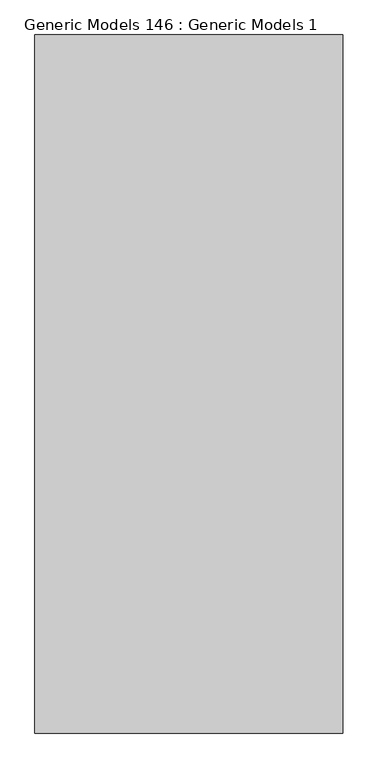
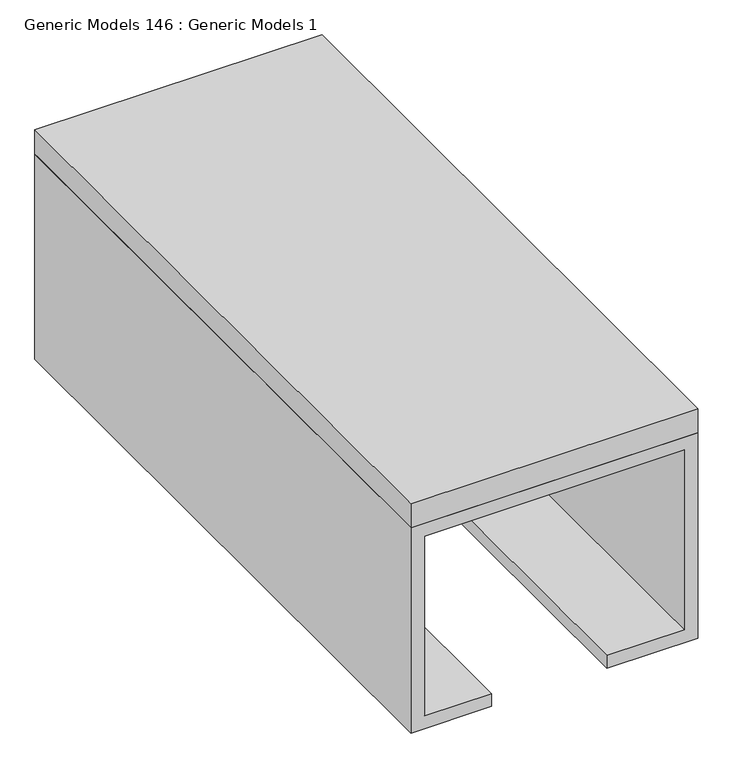
"""IFC4 building model written with IfcOpenShell, lengths in millimetres: proxy geometry, Generic Models 146 : Generic Models 1."""

from ifc_helpers import new_model, si_unit, frame, origin, place, context, project, spatial, polyline, outline, extrude, source, transform, mapped, element, save


def generic_models_146_generic_models_1_9775dfd0(model_context):
    return source(origin(), model_context, "Body", "SweptSolid", [
        extrude(outline(polyline([(51176.9547769, 0.0), (50639.5319345, 0.0), (50639.5319345, 1219.2), (51176.9547769, 1219.2), (51176.9547769, 0.0)])), frame((0.0, 0.0, 2410.0107871), z_axis=(0.0, 0.0, 1.0), x_axis=(1.0, 0.0, 0.0)), (0.0, 0.0, 1.0), 47.4392129),
        extrude(outline(polyline([(2028.825, 50664.9319345), (2384.425, 50664.9319345), (2384.425, 51151.5547769), (2028.825, 51151.5547769), (2028.825, 51006.375), (2003.425, 51006.375), (2003.425, 51176.9547769), (2409.825, 51176.9547769), (2409.825, 50639.5319345), (2003.425, 50639.5319345), (2003.425, 50790.475), (2028.825, 50790.475), (2028.825, 50664.9319345)])), frame((0.0, 0.0, 0.0), z_axis=(0.0, 1.0, 0.0), x_axis=(0.0, 0.0, 1.0)), (0.0, 0.0, 1.0), 1219.2),
    ])


if __name__ == "__main__":
    model = new_model("IFC4")
    model_context = context("Model", 3, world=origin())
    ifc_project = project(units=[si_unit("LENGTHUNIT", "METRE", prefix="MILLI")], contexts=[model_context])
    site = spatial("IfcSite", under=ifc_project)
    building = spatial("IfcBuilding", under=site)
    placement = place(None, origin())
    generic_models_146_generic_models_1_shape = generic_models_146_generic_models_1_9775dfd0(model_context)
    element("IfcBuildingElementProxy", 1, Name="Generic Models 146 : Generic Models 1", ObjectType="Generic Models 146 : Generic Models 1", at=placement, inside=building, context=model_context, shape_type="MappedRepresentation", body=[
        mapped(generic_models_146_generic_models_1_shape, transform((0.0, 0.0, 0.0), x_axis=(1.0, 0.0, 0.0), y_axis=(0.0, 1.0, 0.0), z_axis=(0.0, 0.0, 1.0))),
    ])
    save(model, "model.ifc")

# Revit data of these elements
# Element 1 (IfcBuildingElementProxy, "Generic Models 146 : Generic Models 1")
#   Materials on its faces: "ACOUSTICAL SOUND BARRIER"
# Materials
#   "ACOUSTICAL SOUND BARRIER": class "Generic", colour RGB 215 215 215, transparency 0, Cost = 0
